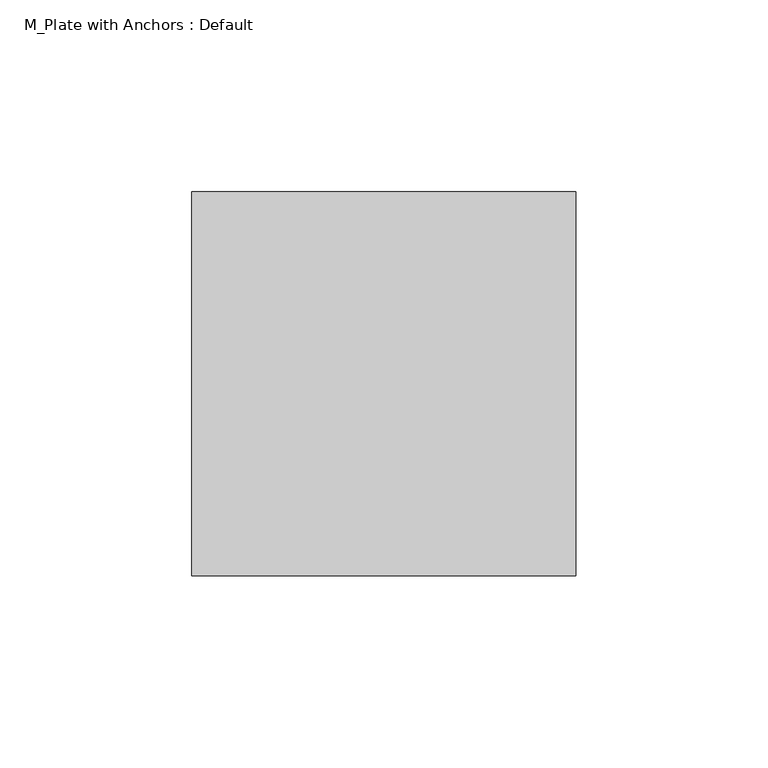
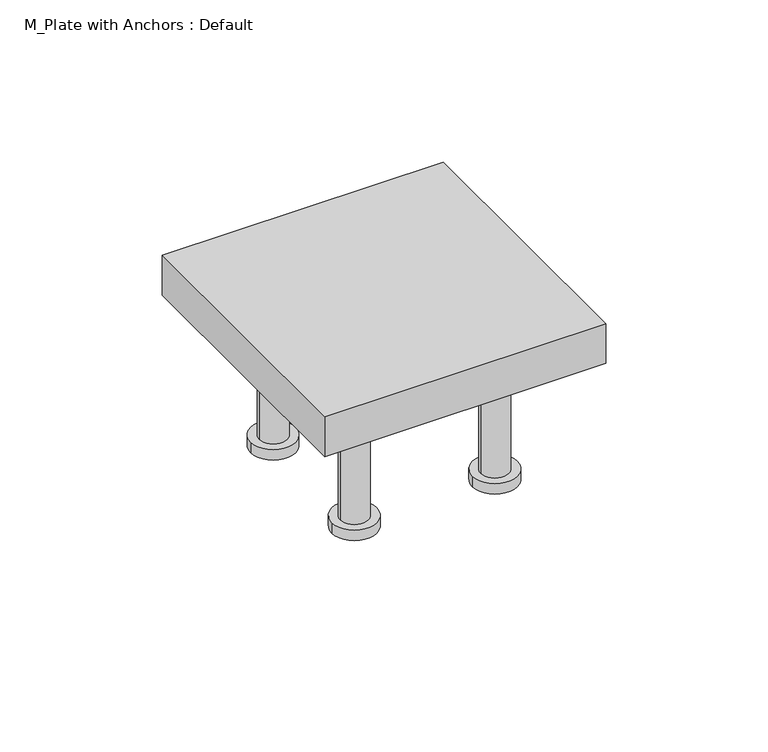
"""IFC4 building model written with IfcOpenShell, lengths in millimetres: fastener geometry, M_Plate with Anchors : Default."""

from ifc_helpers import new_model, si_unit, frame, origin, place, context, project, spatial, polyline, circle_curve, outline, extrude, source, transform, mapped, element, save
from ifc_brep_helpers import plane_surface, cylinder_surface, advanced_brep


def m_plate_with_anchors_default_136118f8(model_context):
    return source(origin(), model_context, "Body", "SolidModel", [
        advanced_brep(
        [(17.0, -25.0, -65.0), (33.0, -25.0, -65.0), (17.0, -25.0, -61.0), (33.0, -25.0, -61.0), (20.0, -25.0, -61.0), (30.0, -25.0, -61.0), (20.0, -25.0, -15.0), (30.0, -25.0, -15.0)],
        [
            (0, 1, circle_curve(frame((25.0, -25.0, -65.0), z_axis=(0.0, 0.0, -1.0), x_axis=(1.0, 0.0, 0.0)), 8.0)),
            (1, 0, circle_curve(frame((25.0, -25.0, -65.0), z_axis=(0.0, 0.0, -1.0), x_axis=(1.0, 0.0, 0.0)), 8.0)),
            (2, 3, circle_curve(frame((25.0, -25.0, -61.0), z_axis=(0.0, 0.0, 1.0), x_axis=(1.0, 0.0, 0.0)), 8.0)),
            (3, 2, circle_curve(frame((25.0, -25.0, -61.0), z_axis=(0.0, 0.0, 1.0), x_axis=(1.0, 0.0, 0.0)), 8.0)),
            (4, 5, circle_curve(frame((25.0, -25.0, -61.0), z_axis=(0.0, 0.0, -1.0), x_axis=(1.0, 0.0, 0.0)), 5.0)),
            (5, 4, circle_curve(frame((25.0, -25.0, -61.0), z_axis=(0.0, 0.0, -1.0), x_axis=(1.0, 0.0, 0.0)), 5.0)),
            (0, 2),
            (3, 1),
            (6, 7, circle_curve(frame((25.0, -25.0, -15.0), z_axis=(0.0, 0.0, 1.0), x_axis=(1.0, 0.0, 0.0)), 5.0)),
            (7, 6, circle_curve(frame((25.0, -25.0, -15.0), z_axis=(0.0, 0.0, 1.0), x_axis=(1.0, 0.0, 0.0)), 5.0)),
            (7, 5),
            (4, 6),
        ],
        [
            plane_surface(frame((33.0, -25.0, -65.0), z_axis=(0.0, 0.0, -1.0), x_axis=(0.0, -1.0, 0.0))),
            plane_surface(frame((33.0, -25.0, -61.0), z_axis=(0.0, 0.0, 1.0), x_axis=(0.0, 1.0, 0.0))),
            cylinder_surface(frame((25.0, -25.0, -61.0), z_axis=(0.0, 0.0, -1.0), x_axis=(1.0, 0.0, 0.0)), 8.0),
            plane_surface(frame((30.0, -25.0, -15.0), z_axis=(0.0, 0.0, 1.0), x_axis=(0.0, 1.0, 0.0))),
            cylinder_surface(frame((25.0, -25.0, -15.0), z_axis=(0.0, 0.0, -1.0), x_axis=(1.0, 0.0, 0.0)), 5.0),
        ],
        [
            (0, [[1, 2]]),
            (1, [[3, 4], [5, 6]]),
            (2, [[-1, 7, -4, 8]]),
            (2, [[-2, -8, -3, -7]]),
            (3, [[9, 10]]),
            (4, [[-10, 11, -5, 12]]),
            (4, [[-9, -12, -6, -11]]),
        ],
    ),
        advanced_brep(
        [(-33.0, -25.0, -65.0), (-17.0, -25.0, -65.0), (-33.0, -25.0, -61.0), (-17.0, -25.0, -61.0), (-30.0, -25.0, -61.0), (-20.0, -25.0, -61.0), (-30.0, -25.0, -15.0), (-20.0, -25.0, -15.0)],
        [
            (0, 1, circle_curve(frame((-25.0, -25.0, -65.0), z_axis=(0.0, 0.0, -1.0), x_axis=(1.0, 0.0, 0.0)), 8.0)),
            (1, 0, circle_curve(frame((-25.0, -25.0, -65.0), z_axis=(0.0, 0.0, -1.0), x_axis=(1.0, 0.0, 0.0)), 8.0)),
            (2, 3, circle_curve(frame((-25.0, -25.0, -61.0), z_axis=(0.0, 0.0, 1.0), x_axis=(1.0, 0.0, 0.0)), 8.0)),
            (3, 2, circle_curve(frame((-25.0, -25.0, -61.0), z_axis=(0.0, 0.0, 1.0), x_axis=(1.0, 0.0, 0.0)), 8.0)),
            (4, 5, circle_curve(frame((-25.0, -25.0, -61.0), z_axis=(0.0, 0.0, -1.0), x_axis=(1.0, 0.0, 0.0)), 5.0)),
            (5, 4, circle_curve(frame((-25.0, -25.0, -61.0), z_axis=(0.0, 0.0, -1.0), x_axis=(1.0, 0.0, 0.0)), 5.0)),
            (0, 2),
            (3, 1),
            (6, 7, circle_curve(frame((-25.0, -25.0, -15.0), z_axis=(0.0, 0.0, 1.0), x_axis=(1.0, 0.0, 0.0)), 5.0)),
            (7, 6, circle_curve(frame((-25.0, -25.0, -15.0), z_axis=(0.0, 0.0, 1.0), x_axis=(1.0, 0.0, 0.0)), 5.0)),
            (7, 5),
            (4, 6),
        ],
        [
            plane_surface(frame((-17.0, -25.0, -65.0), z_axis=(0.0, 0.0, -1.0), x_axis=(0.0, -1.0, 0.0))),
            plane_surface(frame((-17.0, -25.0, -61.0), z_axis=(0.0, 0.0, 1.0), x_axis=(0.0, 1.0, 0.0))),
            cylinder_surface(frame((-25.0, -25.0, -61.0), z_axis=(0.0, 0.0, -1.0), x_axis=(1.0, 0.0, 0.0)), 8.0),
            plane_surface(frame((-20.0, -25.0, -15.0), z_axis=(0.0, 0.0, 1.0), x_axis=(0.0, 1.0, 0.0))),
            cylinder_surface(frame((-25.0, -25.0, -15.0), z_axis=(0.0, 0.0, -1.0), x_axis=(1.0, 0.0, 0.0)), 5.0),
        ],
        [
            (0, [[1, 2]]),
            (1, [[3, 4], [5, 6]]),
            (2, [[-1, 7, -4, 8]]),
            (2, [[-2, -8, -3, -7]]),
            (3, [[9, 10]]),
            (4, [[-10, 11, -5, 12]]),
            (4, [[-9, -12, -6, -11]]),
        ],
    ),
        advanced_brep(
        [(17.0, 25.0, -65.0), (33.0, 25.0, -65.0), (17.0, 25.0, -61.0), (33.0, 25.0, -61.0), (20.0, 25.0, -61.0), (30.0, 25.0, -61.0), (20.0, 25.0, -15.0), (30.0, 25.0, -15.0)],
        [
            (0, 1, circle_curve(frame((25.0, 25.0, -65.0), z_axis=(0.0, 0.0, -1.0), x_axis=(1.0, 0.0, 0.0)), 8.0)),
            (1, 0, circle_curve(frame((25.0, 25.0, -65.0), z_axis=(0.0, 0.0, -1.0), x_axis=(1.0, 0.0, 0.0)), 8.0)),
            (2, 3, circle_curve(frame((25.0, 25.0, -61.0), z_axis=(0.0, 0.0, 1.0), x_axis=(1.0, 0.0, 0.0)), 8.0)),
            (3, 2, circle_curve(frame((25.0, 25.0, -61.0), z_axis=(0.0, 0.0, 1.0), x_axis=(1.0, 0.0, 0.0)), 8.0)),
            (4, 5, circle_curve(frame((25.0, 25.0, -61.0), z_axis=(0.0, 0.0, -1.0), x_axis=(1.0, 0.0, 0.0)), 5.0)),
            (5, 4, circle_curve(frame((25.0, 25.0, -61.0), z_axis=(0.0, 0.0, -1.0), x_axis=(1.0, 0.0, 0.0)), 5.0)),
            (0, 2),
            (3, 1),
            (6, 7, circle_curve(frame((25.0, 25.0, -15.0), z_axis=(0.0, 0.0, 1.0), x_axis=(1.0, 0.0, 0.0)), 5.0)),
            (7, 6, circle_curve(frame((25.0, 25.0, -15.0), z_axis=(0.0, 0.0, 1.0), x_axis=(1.0, 0.0, 0.0)), 5.0)),
            (7, 5),
            (4, 6),
        ],
        [
            plane_surface(frame((33.0, 25.0, -65.0), z_axis=(0.0, 0.0, -1.0), x_axis=(0.0, -1.0, 0.0))),
            plane_surface(frame((33.0, 25.0, -61.0), z_axis=(0.0, 0.0, 1.0), x_axis=(0.0, 1.0, 0.0))),
            cylinder_surface(frame((25.0, 25.0, -61.0), z_axis=(0.0, 0.0, -1.0), x_axis=(1.0, 0.0, 0.0)), 8.0),
            plane_surface(frame((30.0, 25.0, -15.0), z_axis=(0.0, 0.0, 1.0), x_axis=(0.0, 1.0, 0.0))),
            cylinder_surface(frame((25.0, 25.0, -15.0), z_axis=(0.0, 0.0, -1.0), x_axis=(1.0, 0.0, 0.0)), 5.0),
        ],
        [
            (0, [[1, 2]]),
            (1, [[3, 4], [5, 6]]),
            (2, [[-1, 7, -4, 8]]),
            (2, [[-2, -8, -3, -7]]),
            (3, [[9, 10]]),
            (4, [[-10, 11, -5, 12]]),
            (4, [[-9, -12, -6, -11]]),
        ],
    ),
        advanced_brep(
        [(-33.0, 25.0, -65.0), (-17.0, 25.0, -65.0), (-33.0, 25.0, -61.0), (-17.0, 25.0, -61.0), (-30.0, 25.0, -61.0), (-20.0, 25.0, -61.0), (-30.0, 25.0, -15.0), (-20.0, 25.0, -15.0)],
        [
            (0, 1, circle_curve(frame((-25.0, 25.0, -65.0), z_axis=(0.0, 0.0, -1.0), x_axis=(1.0, 0.0, 0.0)), 8.0)),
            (1, 0, circle_curve(frame((-25.0, 25.0, -65.0), z_axis=(0.0, 0.0, -1.0), x_axis=(1.0, 0.0, 0.0)), 8.0)),
            (2, 3, circle_curve(frame((-25.0, 25.0, -61.0), z_axis=(0.0, 0.0, 1.0), x_axis=(1.0, 0.0, 0.0)), 8.0)),
            (3, 2, circle_curve(frame((-25.0, 25.0, -61.0), z_axis=(0.0, 0.0, 1.0), x_axis=(1.0, 0.0, 0.0)), 8.0)),
            (4, 5, circle_curve(frame((-25.0, 25.0, -61.0), z_axis=(0.0, 0.0, -1.0), x_axis=(1.0, 0.0, 0.0)), 5.0)),
            (5, 4, circle_curve(frame((-25.0, 25.0, -61.0), z_axis=(0.0, 0.0, -1.0), x_axis=(1.0, 0.0, 0.0)), 5.0)),
            (0, 2),
            (3, 1),
            (6, 7, circle_curve(frame((-25.0, 25.0, -15.0), z_axis=(0.0, 0.0, 1.0), x_axis=(1.0, 0.0, 0.0)), 5.0)),
            (7, 6, circle_curve(frame((-25.0, 25.0, -15.0), z_axis=(0.0, 0.0, 1.0), x_axis=(1.0, 0.0, 0.0)), 5.0)),
            (7, 5),
            (4, 6),
        ],
        [
            plane_surface(frame((-17.0, 25.0, -65.0), z_axis=(0.0, 0.0, -1.0), x_axis=(0.0, -1.0, 0.0))),
            plane_surface(frame((-17.0, 25.0, -61.0), z_axis=(0.0, 0.0, 1.0), x_axis=(0.0, 1.0, 0.0))),
            cylinder_surface(frame((-25.0, 25.0, -61.0), z_axis=(0.0, 0.0, -1.0), x_axis=(1.0, 0.0, 0.0)), 8.0),
            plane_surface(frame((-20.0, 25.0, -15.0), z_axis=(0.0, 0.0, 1.0), x_axis=(0.0, 1.0, 0.0))),
            cylinder_surface(frame((-25.0, 25.0, -15.0), z_axis=(0.0, 0.0, -1.0), x_axis=(1.0, 0.0, 0.0)), 5.0),
        ],
        [
            (0, [[1, 2]]),
            (1, [[3, 4], [5, 6]]),
            (2, [[-1, 7, -4, 8]]),
            (2, [[-2, -8, -3, -7]]),
            (3, [[9, 10]]),
            (4, [[-10, 11, -5, 12]]),
            (4, [[-9, -12, -6, -11]]),
        ],
    ),
        extrude(outline(polyline([(50.0, 50.0), (50.0, -50.0), (-50.0, -50.0), (-50.0, 50.0), (50.0, 50.0)])), frame((0.0, 0.0, -15.0), z_axis=(0.0, 0.0, 1.0), x_axis=(1.0, 0.0, 0.0)), (0.0, 0.0, 1.0), 15.0),
    ])


if __name__ == "__main__":
    model = new_model("IFC4")
    model_context = context("Model", 3, world=origin())
    ifc_project = project(units=[si_unit("LENGTHUNIT", "METRE", prefix="MILLI")], contexts=[model_context])
    site = spatial("IfcSite", under=ifc_project)
    building = spatial("IfcBuilding", under=site)
    placement = place(None, origin())
    m_plate_with_anchors_default_shape = m_plate_with_anchors_default_136118f8(model_context)
    element("IfcFastener", 1, ObjectType="M_Plate with Anchors : Default", at=placement, inside=building, context=model_context, shape_type="MappedRepresentation", body=[
        mapped(m_plate_with_anchors_default_shape, transform((0.0, 0.0, 0.0), x_axis=(1.0, 0.0, 0.0), y_axis=(0.0, 1.0, 0.0), z_axis=(0.0, 0.0, 1.0))),
    ])
    save(model, "model.ifc")

# Revit data of these elements
# Type "M_Plate with Anchors : Default"
#   Type Comments = "Mountingpart"
#   Plate Width [instance default] = 100 mm
#   Plate Thickness [instance default] = 15 mm
#   Head Radius = 8 mm
#   Rod Radius = 5 mm
#   Plate Length [instance default] = 100 mm
#   Hole Spacing Vertical [instance default] = 50 mm
#   Hole Spacing Horizontal [instance default] = 50 mm
#   Anchor Length [instance default] = 50 mm
#   Number of Bolts [instance default] = 2
#   Plate Material [instance default] = Metal - Steel - S235
#   Anchor Material [instance default] = Metal - Steel - S235
#   Default Elevation = 0
# Element 1 (IfcFastener, "M_Plate with Anchors : Default")
#   Materials on its faces: "Metal - Steel - S235"
# Materials
#   "Metal - Steel - S235": class "Steel", colour RGB 247 247 247, transparency 0, Cost = 0
